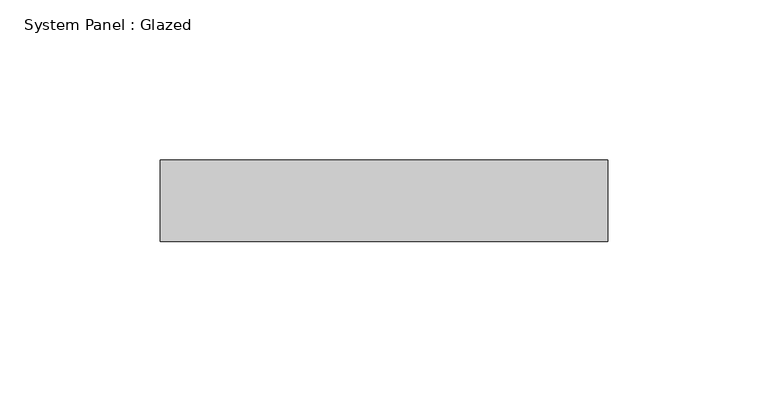
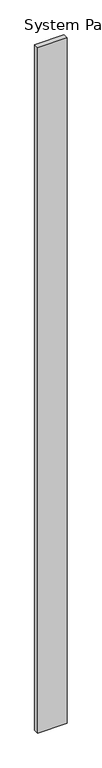
"""IFC4 building model written with IfcOpenShell, lengths in millimetres: plate geometry, System Panel : Glazed."""

import ifcopenshell
import ifcopenshell.guid

model = None  # the IFC model being written
_history = None  # IfcOwnerHistory: only IFC2X3 demands one
_inside = {}  # id of a spatial element -> (the spatial element, [elements in it])
_under = {}  # id of a project, library or spatial element -> (it, [spatial elements below it])
_declared = {}  # id of a project -> (the project, [libraries it declares])
_typed = {}  # id of a type object -> (the type object, [elements of that type])
_made_of = {}  # id of a material, layer set ... -> (it, [elements and type objects made of it])


def new_model(schema):
    """Start an empty IFC model of exactly this schema.

    Asked for "IFC4X3", IfcOpenShell would pick the latest addendum, in which some entities
    have other attributes; the version numbers below select the first issue.
    IFC2X3 requires an IfcOwnerHistory on every rooted entity: one is made here for all.
    """
    global model, _history
    if schema == "IFC4X3":
        model = ifcopenshell.file(schema_version=(4, 3, 0, 0))
    else:
        model = ifcopenshell.file(schema=schema)
    _inside.clear()
    _under.clear()
    _declared.clear()
    _typed.clear()
    _made_of.clear()
    _history = None
    if model.schema == "IFC2X3":
        org = make("IfcOrganization", Name="unknown")
        user = make(
            "IfcPersonAndOrganization",
            ThePerson=make("IfcPerson", FamilyName="unknown"),
            TheOrganization=org,
        )
        app = make(
            "IfcApplication",
            ApplicationDeveloper=org,
            Version="unknown",
            ApplicationFullName="unknown",
            ApplicationIdentifier="unknown",
        )
        _history = make(
            "IfcOwnerHistory",
            OwningUser=user,
            OwningApplication=app,
            ChangeAction="ADDED",
            CreationDate=0,
        )
    return model


def make(cls, **values):
    """One entity of the class cls with the attributes given. An attribute that is None is left unset."""
    return model.create_entity(
        cls, **{name: value for name, value in values.items() if value is not None}
    )


def rooted(cls, **values):
    """An entity with a GlobalId (a new one), such as an element, a storey or a relation."""
    return make(cls, GlobalId=ifcopenshell.guid.new(), OwnerHistory=_history, **values)


def si_unit(unit_type, name, prefix=None):
    """IfcSIUnit, for example si_unit("LENGTHUNIT", "METRE", prefix="MILLI")."""
    return make("IfcSIUnit", UnitType=unit_type, Prefix=prefix, Name=name)


def assignment(units):
    """IfcUnitAssignment: the units of a project."""
    return None if units is None else make("IfcUnitAssignment", Units=units)


def point(xyz):
    """IfcCartesianPoint."""
    return None if xyz is None else make("IfcCartesianPoint", Coordinates=xyz)


def direction(xyz):
    """IfcDirection."""
    return None if xyz is None else make("IfcDirection", DirectionRatios=xyz)


def frame(location, z_axis=None, x_axis=None):
    """IfcAxis2Placement3D, a coordinate frame: its origin and axes. An axis left out is left unset."""
    return make(
        "IfcAxis2Placement3D",
        Location=point(location),
        Axis=direction(z_axis),
        RefDirection=direction(x_axis),
    )


def origin():
    """The frame at (0, 0, 0) with its axes left unset."""
    return frame((0.0, 0.0, 0.0))


def origin_with_axes():
    """The frame at (0, 0, 0) with the z axis (0, 0, 1) and the x axis (1, 0, 0) written out."""
    return frame((0.0, 0.0, 0.0), z_axis=(0.0, 0.0, 1.0), x_axis=(1.0, 0.0, 0.0))


def place(relative_to, where):
    """IfcLocalPlacement: puts the frame where relative to a parent placement (None: the world)."""
    return make(
        "IfcLocalPlacement", PlacementRelTo=relative_to, RelativePlacement=where
    )


def context(
    kind, dimensions, precision=None, world=None, true_north=None, identifier=None
):
    """IfcGeometricRepresentationContext, for example the 3D "Model" context."""
    return make(
        "IfcGeometricRepresentationContext",
        ContextIdentifier=identifier,
        ContextType=kind,
        CoordinateSpaceDimension=dimensions,
        Precision=precision,
        WorldCoordinateSystem=world,
        TrueNorth=true_north,
    )


def project(units=None, contexts=None):
    """IfcProject with its units and contexts."""
    return rooted(
        "IfcProject",
        Name="project",
        RepresentationContexts=contexts,
        UnitsInContext=assignment(units),
    )


def spatial(cls, under=None, at=None, **own):
    """A site, building, storey or space (cls), placed at a placement, below another one or the project."""
    s = rooted(cls, ObjectPlacement=at, **own)
    if under is not None:
        _under.setdefault(under.id(), (under, []))[1].append(s)
    return s


def polyline(points):
    """IfcPolyline through the points."""
    return make("IfcPolyline", Points=[point(p) for p in points])


def outline(outer, holes=None, kind="AREA"):
    """IfcArbitraryClosedProfileDef: a profile drawn as a closed curve; with holes, ...WithVoids."""
    if holes is None:
        return make("IfcArbitraryClosedProfileDef", ProfileType=kind, OuterCurve=outer)
    return make(
        "IfcArbitraryProfileDefWithVoids",
        ProfileType=kind,
        OuterCurve=outer,
        InnerCurves=holes,
    )


def extrude(swept, where, along, depth):
    """IfcExtrudedAreaSolid: the profile swept, set in the frame where, extruded along a direction by depth."""
    return make(
        "IfcExtrudedAreaSolid",
        SweptArea=swept,
        Position=where,
        ExtrudedDirection=direction(along),
        Depth=depth,
    )


def shape(context_of_items, identifier, shape_type, items):
    """IfcShapeRepresentation: the items that make up one representation, for example the "Body"."""
    return make(
        "IfcShapeRepresentation",
        ContextOfItems=context_of_items,
        RepresentationIdentifier=identifier,
        RepresentationType=shape_type,
        Items=items,
    )


def source(mapping_origin, context_of_items, identifier, shape_type, items):
    """IfcRepresentationMap: a shape defined once, which mapped items show again and again."""
    return make(
        "IfcRepresentationMap",
        MappingOrigin=mapping_origin,
        MappedRepresentation=shape(context_of_items, identifier, shape_type, items),
    )


def transform(
    local_origin,
    x_axis=None,
    y_axis=None,
    z_axis=None,
    scale=None,
    scale2=None,
    scale3=None,
    uniform=True,
):
    """IfcCartesianTransformationOperator3D, or its non-uniform kind. x_axis, y_axis, z_axis: its Axis1, 2, 3."""
    if uniform:
        return make(
            "IfcCartesianTransformationOperator3D",
            Axis1=direction(x_axis),
            Axis2=direction(y_axis),
            LocalOrigin=point(local_origin),
            Scale=scale,
            Axis3=direction(z_axis),
        )
    return make(
        "IfcCartesianTransformationOperator3DnonUniform",
        Axis1=direction(x_axis),
        Axis2=direction(y_axis),
        LocalOrigin=point(local_origin),
        Scale=scale,
        Axis3=direction(z_axis),
        Scale2=scale2,
        Scale3=scale3,
    )


def mapped(mapping_source, mapping_target):
    """IfcMappedItem: shows the shape of a source again, moved by a transform."""
    return make(
        "IfcMappedItem", MappingSource=mapping_source, MappingTarget=mapping_target
    )


def made_of(thing, what):
    """Note that an element or type object is made of a material, layer set ...; save() writes the relation."""
    if what is not None:
        _made_of.setdefault(what.id(), (what, []))[1].append(thing)
    return thing


def element(
    cls,
    number,
    at=None,
    inside=None,
    cuts=None,
    type_object=None,
    material=None,
    context=None,
    identifier="Body",
    shape_type=None,
    held_by="IfcProductDefinitionShape",
    body=None,
    shapes=None,
    **own,
):
    """One element of the class cls, such as IfcWall. Its Tag is "e" and its number.

    at: its placement. inside: the storey or other place that contains it. cuts: it is an
    opening in that element (IfcRelVoidsElement). A single representation is given by context,
    identifier, shape_type and body (its items); several are given by shapes. held_by: the class
    of the entity that holds the representations. save() writes the other relations.
    """
    e = rooted(cls, Tag="e%d" % number, ObjectPlacement=at, **own)
    if body is not None:
        shapes = [shape(context, identifier, shape_type, body)]
    if shapes is not None:
        e.Representation = make(held_by, Representations=shapes)
    if inside is not None:
        _inside.setdefault(inside.id(), (inside, []))[1].append(e)
    if cuts is not None:
        rooted(
            "IfcRelVoidsElement", RelatingBuildingElement=cuts, RelatedOpeningElement=e
        )
    if type_object is not None:
        _typed.setdefault(type_object.id(), (type_object, []))[1].append(e)
    return made_of(e, material)


def aggregate(whole, parts):
    """IfcRelAggregates: a whole, such as a stair, and the parts it consists of."""
    return rooted("IfcRelAggregates", RelatingObject=whole, RelatedObjects=parts)


def save(model, path):
    """Write the relations noted so far, then the file.

    IfcRelAggregates (storeys below a building ...), IfcRelContainedInSpatialStructure (elements
    in a storey), IfcRelDefinesByType, IfcRelAssociatesMaterial and IfcRelDeclares: one each for
    every whole, place, type object, material and project.
    """
    for whole, parts in _under.values():
        aggregate(whole, parts)
    for where, things in _inside.values():
        rooted(
            "IfcRelContainedInSpatialStructure",
            RelatedElements=things,
            RelatingStructure=where,
        )
    for kind, things in _typed.values():
        rooted("IfcRelDefinesByType", RelatedObjects=things, RelatingType=kind)
    for what, things in _made_of.values():
        rooted("IfcRelAssociatesMaterial", RelatedObjects=things, RelatingMaterial=what)
    for by, libraries in _declared.values():
        rooted("IfcRelDeclares", RelatingContext=by, RelatedDefinitions=libraries)
    model.write(path)


def system_panel_glazed_c127a6e8(model_context):
    return source(origin(), model_context, "Body", "SweptSolid", [
        extrude(outline(polyline([(69.649919, 19.05), (-69.649919, 19.05), (-69.649919, 44.45), (69.649919, 44.45), (69.649919, 19.05)])), origin_with_axes(), (0.0, 0.0, 1.0), 3454.4),
    ])


if __name__ == "__main__":
    model = new_model("IFC4")
    model_context = context("Model", 3, world=origin())
    ifc_project = project(units=[si_unit("LENGTHUNIT", "METRE", prefix="MILLI")], contexts=[model_context])
    site = spatial("IfcSite", under=ifc_project)
    building = spatial("IfcBuilding", under=site)
    placement = place(None, origin())
    system_panel_glazed_shape = system_panel_glazed_c127a6e8(model_context)
    element("IfcPlate", 1, ObjectType="System Panel : Glazed", at=placement, inside=building, context=model_context, shape_type="MappedRepresentation", body=[
        mapped(system_panel_glazed_shape, transform((0.0, 0.0, 0.0), x_axis=(1.0, 0.0, 0.0), y_axis=(0.0, 1.0, 0.0), z_axis=(0.0, 0.0, 1.0))),
    ])
    save(model, "model.ifc")

# Revit data of these elements
# Type "System Panel : Glazed"
#   Construction Type Id = "GSP4R"
#   Analytic Construction = "1/8 in Pilkington single glazing"
#   Visual Light Transmittance = 0.9
#   Solar Heat Gain Coefficient = 0.86
#   Heat Transfer Coefficient (U) = 1.18115 BTU/(h·ft²·°F)
#   Define Thermal Properties by = 1
# Element 1 (IfcPlate, "System Panel : Glazed")
#   Materials on its faces: "Glass"
# Materials
#   "Glass": class "Glass", colour RGB 0 128 192, transparency 0.75, Description = "Soda Lime Glass", Cost = 0
